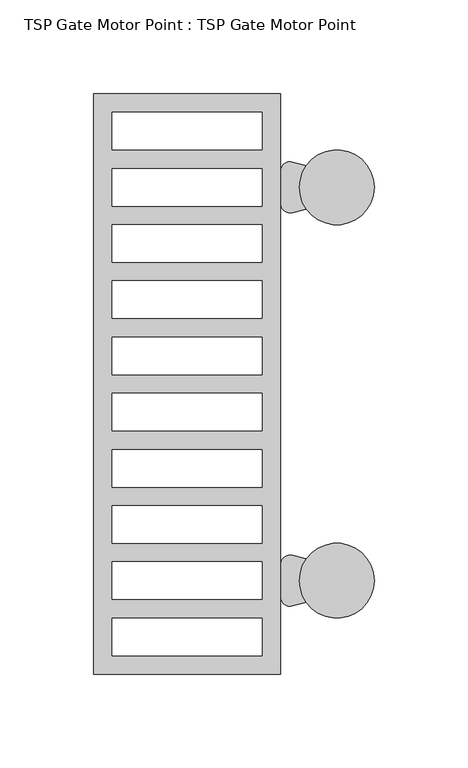
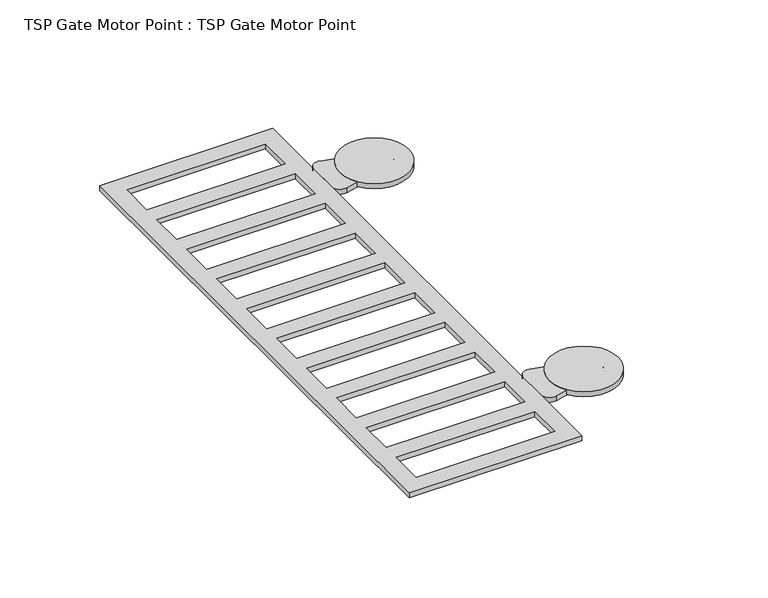
"""IFC4 building model written with IfcOpenShell, lengths in millimetres: proxy geometry, TSP Gate Motor Point : TSP Gate Motor Point."""

from ifc_helpers import new_model, si_unit, point, frame_2d, origin, origin_with_axes, place, context, project, spatial, polyline, circle_curve, trimmed, segment, composite_curve, outline, extrude, source, transform, mapped, element, save


def tsp_gate_motor_point_tsp_gate_motor_point_92d777b9(model_context):
    return source(origin(), model_context, "Body", "SweptSolid", [
        extrude(outline(polyline([(-50.0, 155.0), (-50.0, -155.0), (-150.0, -155.0), (-150.0, 155.0), (-50.0, 155.0)]), holes=[polyline([(-60.0, 5.0), (-60.0, 25.0), (-140.0, 25.0), (-140.0, 5.0), (-60.0, 5.0)]), polyline([(-140.0, -5.0), (-140.0, -25.0), (-60.0, -25.0), (-60.0, -5.0), (-140.0, -5.0)]), polyline([(-60.0, 95.0), (-60.0, 115.0), (-140.0, 115.0), (-140.0, 95.0), (-60.0, 95.0)]), polyline([(-60.0, 125.0), (-60.0, 145.0), (-140.0, 145.0), (-140.0, 125.0), (-60.0, 125.0)]), polyline([(-60.0, -95.0), (-140.0, -95.0), (-140.0, -115.0), (-60.0, -115.0), (-60.0, -95.0)]), polyline([(-60.0, -125.0), (-140.0, -125.0), (-140.0, -145.0), (-60.0, -145.0), (-60.0, -125.0)]), polyline([(-60.0, 65.0), (-60.0, 85.0), (-140.0, 85.0), (-140.0, 65.0), (-60.0, 65.0)]), polyline([(-140.0, 55.0), (-140.0, 35.0), (-60.0, 35.0), (-60.0, 55.0), (-140.0, 55.0)]), polyline([(-60.0, -55.0), (-60.0, -35.0), (-140.0, -35.0), (-140.0, -55.0), (-60.0, -55.0)]), polyline([(-140.0, -65.0), (-140.0, -85.0), (-60.0, -85.0), (-60.0, -65.0), (-140.0, -65.0)])]), origin_with_axes(), (0.0, 0.0, 1.0), 3.0),
        extrude(outline(composite_curve([segment(trimmed(circle_curve(frame_2d((-20.0, 105.0)), 20.0), [point((-40.0, 105.0))], [point((0.0, 105.0))], False, "CARTESIAN"), True, "CONTINUOUS"), segment(trimmed(circle_curve(frame_2d((-20.0, 105.0)), 20.0), [point((0.0, 105.0))], [point((-40.0, 105.0))], False, "CARTESIAN"), True, "CONTINUOUS")], self_intersect=False)), origin_with_axes(), (0.0, 0.0, 1.0), 3.0),
        extrude(outline(composite_curve([segment(trimmed(circle_curve(frame_2d((-20.0, -105.0)), 20.0), [point((-40.0, -105.0))], [point((0.0, -105.0))], False, "CARTESIAN"), True, "CONTINUOUS"), segment(trimmed(circle_curve(frame_2d((-20.0, -105.0)), 20.0), [point((0.0, -105.0))], [point((-40.0, -105.0))], False, "CARTESIAN"), True, "CONTINUOUS")], self_intersect=False)), origin_with_axes(), (0.0, 0.0, 1.0), 3.0),
        extrude(outline(composite_curve([segment(trimmed(circle_curve(frame_2d((-15.0, 103.903882)), 5.0), [point((-10.0, 103.903882))], [point((-13.7873219, 99.0531695))], False, "CARTESIAN"), True, "CONTINUOUS"), segment(polyline([(-13.7873219, 99.0531695), (-43.7873219, 91.5531695)]), True, "CONTINUOUS"), segment(trimmed(circle_curve(frame_2d((-45.0, 96.403882)), 5.0), [point((-43.7873219, 91.5531695))], [point((-50.0, 96.403882))], False, "CARTESIAN"), True, "CONTINUOUS"), segment(polyline([(-50.0, 96.403882), (-50.0, 113.596118)]), True, "CONTINUOUS"), segment(trimmed(circle_curve(frame_2d((-45.0, 113.596118)), 5.0), [point((-50.0, 113.596118))], [point((-43.7873219, 118.4468305))], False, "CARTESIAN"), True, "CONTINUOUS"), segment(polyline([(-43.7873219, 118.4468305), (-13.7873219, 110.9468305)]), True, "CONTINUOUS"), segment(trimmed(circle_curve(frame_2d((-15.0, 106.096118)), 5.0), [point((-13.7873219, 110.9468305))], [point((-10.0, 106.096118))], False, "CARTESIAN"), True, "CONTINUOUS"), segment(polyline([(-10.0, 106.096118), (-10.0, 105.0), (-10.0, 103.903882)]), True, "CONTINUOUS")], self_intersect=False)), origin_with_axes(), (0.0, 0.0, 1.0), 3.0),
        extrude(outline(composite_curve([segment(polyline([(-10.0, -103.903882), (-10.0, -105.0), (-10.0, -106.096118)]), True, "CONTINUOUS"), segment(trimmed(circle_curve(frame_2d((-15.0, -106.096118)), 5.0), [point((-10.0, -106.096118))], [point((-13.7873219, -110.9468305))], False, "CARTESIAN"), True, "CONTINUOUS"), segment(polyline([(-13.7873219, -110.9468305), (-43.7873219, -118.4468305)]), True, "CONTINUOUS"), segment(trimmed(circle_curve(frame_2d((-45.0, -113.596118)), 5.0), [point((-43.7873219, -118.4468305))], [point((-50.0, -113.596118))], False, "CARTESIAN"), True, "CONTINUOUS"), segment(polyline([(-50.0, -113.596118), (-50.0, -96.403882)]), True, "CONTINUOUS"), segment(trimmed(circle_curve(frame_2d((-45.0, -96.403882)), 5.0), [point((-50.0, -96.403882))], [point((-43.7873219, -91.5531695))], False, "CARTESIAN"), True, "CONTINUOUS"), segment(polyline([(-43.7873219, -91.5531695), (-13.7873219, -99.0531695)]), True, "CONTINUOUS"), segment(trimmed(circle_curve(frame_2d((-15.0, -103.903882)), 5.0), [point((-13.7873219, -99.0531695))], [point((-10.0, -103.903882))], False, "CARTESIAN"), True, "CONTINUOUS")], self_intersect=False)), origin_with_axes(), (0.0, 0.0, 1.0), 3.0),
    ])


if __name__ == "__main__":
    model = new_model("IFC4")
    model_context = context("Model", 3, world=origin())
    ifc_project = project(units=[si_unit("LENGTHUNIT", "METRE", prefix="MILLI")], contexts=[model_context])
    site = spatial("IfcSite", under=ifc_project)
    building = spatial("IfcBuilding", under=site)
    placement = place(None, origin())
    tsp_gate_motor_point_tsp_gate_motor_point_shape = tsp_gate_motor_point_tsp_gate_motor_point_92d777b9(model_context)
    element("IfcBuildingElementProxy", 1, Name="TSP Gate Motor Point : TSP Gate Motor Point", ObjectType="TSP Gate Motor Point : TSP Gate Motor Point", at=placement, inside=building, context=model_context, shape_type="MappedRepresentation", body=[
        mapped(tsp_gate_motor_point_tsp_gate_motor_point_shape, transform((0.0, 0.0, 0.0), x_axis=(1.0, 0.0, 0.0), y_axis=(0.0, 1.0, 0.0), z_axis=(0.0, 0.0, 1.0))),
    ])
    save(model, "model.ifc")

# Revit data of these elements
# Type "TSP Gate Motor Point : TSP Gate Motor Point"
#   Model = "TSP_ELECEGMP"
#   Default Elevation = 0
# Element 1 (IfcBuildingElementProxy, "TSP Gate Motor Point : TSP Gate Motor Point")
#   Materials on its faces: "Plastic, Opaque Black"
# Materials
#   "Plastic, Opaque Black": class "Plastic", colour RGB 0 0 0, transparency 0.7, Description = "Plastic, generic, opaque black", Cost = 0
